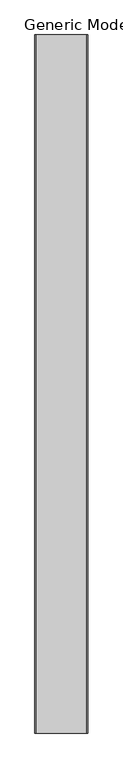
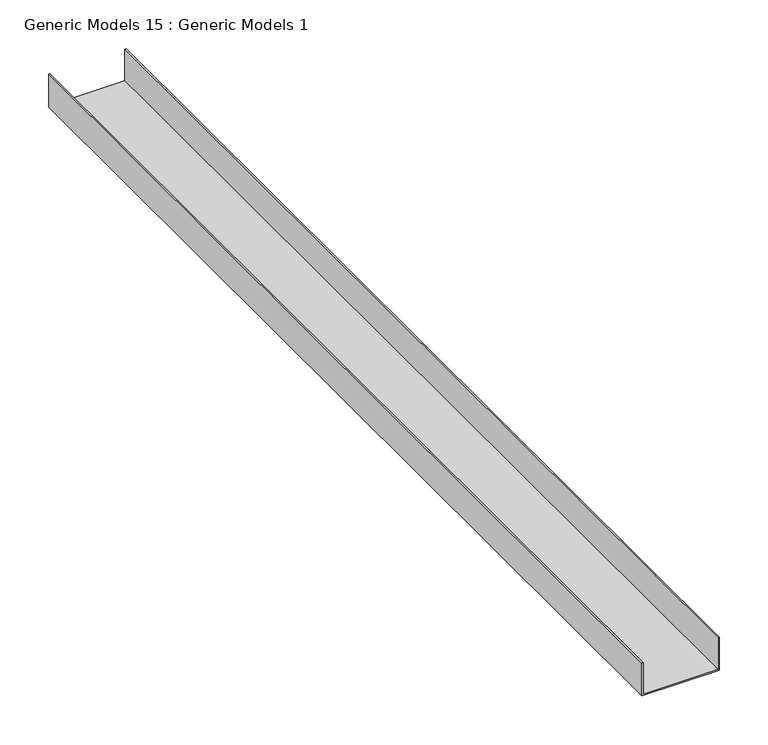
"""IFC4 building model written with IfcOpenShell, lengths in millimetres: proxy geometry, Generic Models 15 : Generic Models 1."""

from ifc_helpers import new_model, si_unit, frame, origin, place, context, project, spatial, polyline, outline, extrude, source, transform, mapped, element, save


def generic_models_15_generic_models_1_38d4618c(model_context):
    return source(origin(), model_context, "Body", "SweptSolid", [
        extrude(outline(polyline([(0.0, 49784.0), (41.275, 49784.0), (41.275, 49782.4125), (1.5875, 49782.4125), (1.5875, 49693.5125), (41.275, 49693.5125), (41.275, 49691.925), (0.0, 49691.925), (0.0, 49784.0)])), frame((0.0, 0.0, 0.0), z_axis=(0.0, 1.0, 0.0), x_axis=(0.0, 0.0, 1.0)), (0.0, 0.0, 1.0), 1219.2),
    ])


if __name__ == "__main__":
    model = new_model("IFC4")
    model_context = context("Model", 3, world=origin())
    ifc_project = project(units=[si_unit("LENGTHUNIT", "METRE", prefix="MILLI")], contexts=[model_context])
    site = spatial("IfcSite", under=ifc_project)
    building = spatial("IfcBuilding", under=site)
    placement = place(None, origin())
    generic_models_15_generic_models_1_shape = generic_models_15_generic_models_1_38d4618c(model_context)
    element("IfcBuildingElementProxy", 1, Name="Generic Models 15 : Generic Models 1", ObjectType="Generic Models 15 : Generic Models 1", at=placement, inside=building, context=model_context, shape_type="MappedRepresentation", body=[
        mapped(generic_models_15_generic_models_1_shape, transform((0.0, 0.0, 0.0), x_axis=(1.0, 0.0, 0.0), y_axis=(0.0, 1.0, 0.0), z_axis=(0.0, 0.0, 1.0))),
    ])
    save(model, "model.ifc")

# Revit data of these elements
# Element 1 (IfcBuildingElementProxy, "Generic Models 15 : Generic Models 1")
#   Materials on its faces: "METAL RUNNER CHANNEL; FASTEN @ 24\" O.C."
# Materials
#   "METAL RUNNER CHANNEL; FASTEN @ 24\" O.C.": class "Unassigned", colour RGB 210 209 208, transparency 0, Keynote = "M05121300.02", Cost = 0
